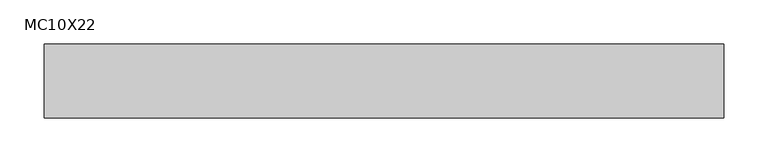
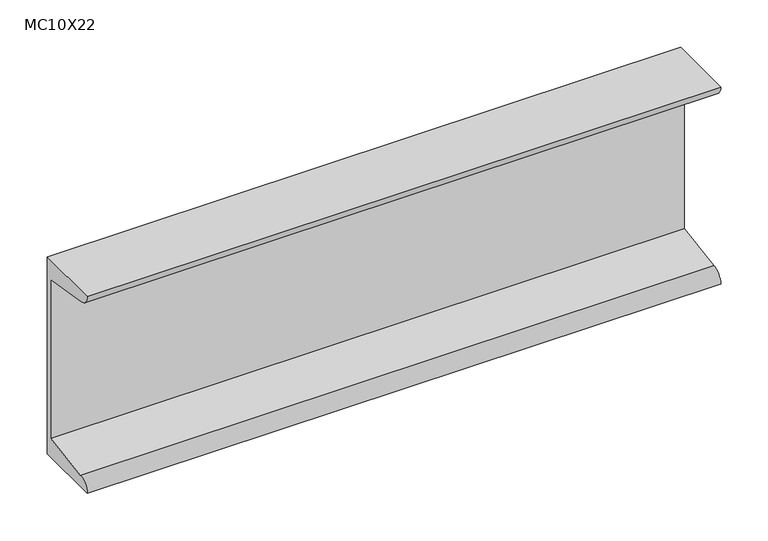
"""IFC4 building model written with IfcOpenShell, lengths in millimetres: beam geometry, MC-Miscellaneous Channel : MC10X22."""

from ifc_helpers import new_model, si_unit, point, frame, frame_2d, origin, place, context, project, spatial, polyline, circle_curve, trimmed, segment, composite_curve, outline, extrude, source, transform, mapped, element, save


def mc10x22_943ffe2d(model_context):
    return source(origin(), model_context, "Body", "SweptSolid", [
        extrude(outline(composite_curve([segment(polyline([(25.146, 127.0), (25.146, -127.0), (-59.182, -127.0)]), True, "CONTINUOUS"), segment(trimmed(circle_curve(frame_2d((-44.577, -127.0)), 14.605), [point((-59.182, -127.0))], [point((-44.577, -112.395))], False, "CARTESIAN"), True, "CONTINUOUS"), segment(polyline([(-44.577, -112.395), (17.78, -102.5186215), (17.78, 102.5186215), (-44.577, 112.395)]), True, "CONTINUOUS"), segment(trimmed(circle_curve(frame_2d((-44.577, 127.0)), 14.605), [point((-44.577, 112.395))], [point((-59.182, 127.0))], False, "CARTESIAN"), True, "CONTINUOUS"), segment(polyline([(-59.182, 127.0), (25.146, 127.0)]), True, "CONTINUOUS")], self_intersect=False)), frame((-386.1670251, 0.0, 0.0), z_axis=(1.0, 0.0, 0.0), x_axis=(0.0, 1.0, 0.0)), (0.0, 0.0, 1.0), 772.3340502),
    ])


if __name__ == "__main__":
    model = new_model("IFC4")
    model_context = context("Model", 3, world=origin())
    ifc_project = project(units=[si_unit("LENGTHUNIT", "METRE", prefix="MILLI")], contexts=[model_context])
    site = spatial("IfcSite", under=ifc_project)
    building = spatial("IfcBuilding", under=site)
    placement = place(None, origin())
    mc10x22_shape = mc10x22_943ffe2d(model_context)
    element("IfcBeam", 1, ObjectType="MC-Miscellaneous Channel : MC10X22", at=placement, inside=building, context=model_context, shape_type="MappedRepresentation", body=[
        mapped(mc10x22_shape, transform((0.0, 0.0, 0.0), x_axis=(1.0, 0.0, 0.0), y_axis=(0.0, 1.0, 0.0), z_axis=(0.0, 0.0, 1.0))),
    ])
    save(model, "model.ifc")

# Revit data of these elements
# Type "MC-Miscellaneous Channel : MC10X22"
#   Assembly Code = "B10"
#   W = 22
#   Length [instance default] = 5' - 0"
#   bf = 0' - 3.32"
#   d = 0' - 10"
#   tf = 0' - 0.575"
#   tw = 0' - 0.29"
#   x = 0' - 0.99"
#   A = 0.0447917 SF
#   Structural Material [instance default] = Steel ASTM A36
# Element 1 (IfcBeam, "MC-Miscellaneous Channel : MC10X22")
#   Length = 2' - 6.40685"
#   Structural Material = Metal - Steel - ASTM A992
#   Materials on its faces: "Metal - Steel - ASTM A992"
# Materials
#   "Steel ASTM A36": class "Metal", colour RGB 199 199 199, transparency 0, Description = "Structural steel, ASTM A36 Grade B, mill finish", Cost = 0
#   "Metal - Steel - ASTM A992": class "Metal", colour RGB 255 128 0, transparency 0
